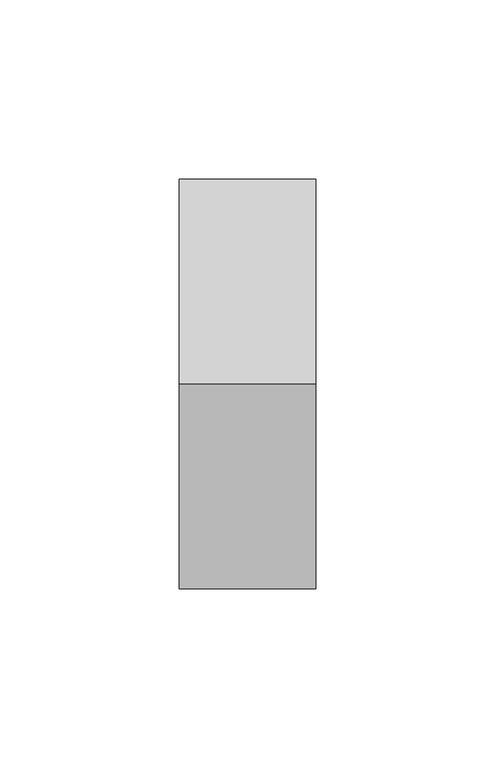
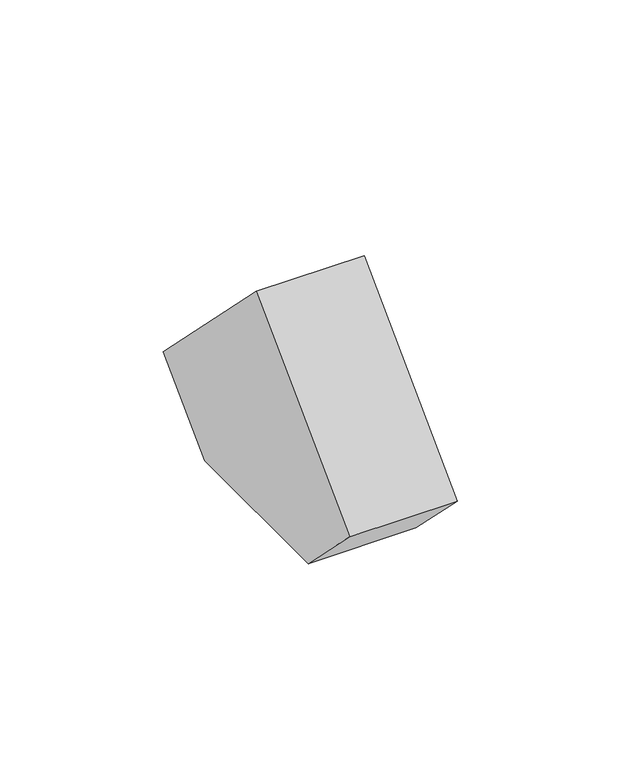
"""IFC4 building model written with IfcOpenShell, lengths in millimetres: proxy geometry, Inner panel:Inner panel:1:Inner panel:1 : Inner panel:Inner panel:300324:2:Inner panel:1:Inner panel:1 : Inner panel:Inner panel:300324:2 : Inner panel:Inner panel:1:Inner panel:1 : Inner panel:Inner panel:300324:300043:2 : Inner panel:Inner panel:1:Inner panel:1 : Inner panel:Inner panel:300324:2:Inner panel:1:Inner panel:1 : Inner panel:Inner panel:300324:2 : Inner panel:Inner panel:1:Inner panel:1 : Inner panel:Inner panel:300324:300043:308120."""

from ifc_helpers import new_model, si_unit, frame, origin, place, context, project, spatial, polyline, outline, extrude, source, transform, mapped, element, save


def generic_models_094954bc(model_context):
    return source(origin(), model_context, "Body", "SweptSolid", [
        extrude(outline(polyline([(-569594.8513281, 8849.4498692), (-569620.2513282, 8824.0498691), (-569683.7513282, 8824.0498691), (-569709.1513281, 8849.4498691), (-569652.0013281, 8906.5998691), (-569594.8513281, 8849.4498692)])), frame((593426.9367239, 0.0, 0.0), z_axis=(1.0, 0.0, 0.0), x_axis=(0.0, 1.0, 0.0)), (0.0, 0.0, 1.0), 38.1),
    ])


if __name__ == "__main__":
    model = new_model("IFC4")
    model_context = context("Model", 3, world=origin())
    ifc_project = project(units=[si_unit("LENGTHUNIT", "METRE", prefix="MILLI")], contexts=[model_context])
    site = spatial("IfcSite", under=ifc_project)
    building = spatial("IfcBuilding", under=site)
    placement = place(None, origin())
    generic_models_shape = generic_models_094954bc(model_context)
    element("IfcBuildingElementProxy", 1, Name="Inner panel:Inner panel:1:Inner panel:1 : Inner panel:Inner panel:300324:2:Inner panel:1:Inner panel:1 : Inner panel:Inner panel:300324:2 : Inner panel:Inner panel:1:Inner panel:1 : Inner panel:Inner panel:300324:300043:2 : Inner panel:Inner panel:1:Inner panel:1 : Inner panel:Inner panel:300324:2:Inner panel:1:Inner panel:1 : Inner panel:Inner panel:300324:2 : Inner panel:Inner panel:1:Inner panel:1 : Inner panel:Inner panel:300324:300043:308120", ObjectType="Inner panel:Inner panel:1:Inner panel:1 : Inner panel:Inner panel:300324:2:Inner panel:1:Inner panel:1 : Inner panel:Inner panel:300324:2 : Inner panel:Inner panel:1:Inner panel:1 : Inner panel:Inner panel:300324:300043:2 : Inner panel:Inner panel:1:Inner panel:1 : Inner panel:Inner panel:300324:2:Inner panel:1:Inner panel:1 : Inner panel:Inner panel:300324:2 : Inner panel:Inner panel:1:Inner panel:1 : Inner panel:Inner panel:300324:300043:308120", at=placement, inside=building, context=model_context, shape_type="MappedRepresentation", body=[
        mapped(generic_models_shape, transform((0.0, 0.0, 0.0), x_axis=(1.0, 0.0, 0.0), y_axis=(0.0, 1.0, 0.0), z_axis=(0.0, 0.0, 1.0))),
    ])
    save(model, "model.ifc")

# Revit data of these elements
# Type "Inner panel:Inner panel:1:Inner panel:1 : Inner panel:Inner panel:300324:2:Inner panel:1:Inner panel:1 : Inner panel:Inner panel:300324:2 : Inner panel:Inner panel:1:Inner panel:1 : Inner panel:Inner panel:300324:300043:2 : Inner panel:Inner panel:1:Inner panel:1 : Inner panel:Inner panel:300324:2:Inner panel:1:Inner panel:1 : Inner panel:Inner panel:300324:2 : Inner panel:Inner panel:1:Inner panel:1 : Inner panel:Inner panel:300324:300043:308120"
#   NameOverride = "Inner panel:Inner panel:1:Inner panel:1 : Inner panel:Inner panel:300324:2:Inner panel:1:Inner panel:1 : Inner panel:Inner panel:300324:2 : Inner panel:Inner panel:1:Inner panel:1 : Inner panel:Inner panel:300324:300043:308120"
#   ObjectTypeOverride = "Inner panel:1:Inner panel:1 : Inner panel:Inner panel:300324:2 : Inner panel:Inner panel:1:Inner panel:1 : Inner panel:Inner panel:300324:300043"
#   Reference = "Inner panel"
#   Tag = "308120"
# Element 1 (IfcBuildingElementProxy, "Inner panel:Inner panel:1:Inner panel:1 : Inner panel:Inner panel:300324:2:Inner panel:1:Inner panel:1 : Inner panel:Inner panel:300324:2 : Inner panel:Inner panel:1:Inner panel:1 : Inner panel:Inner panel:300324:300043:2 : Inner panel:Inner panel:1:Inner panel:1 : Inner panel:Inner panel:300324:2:Inner panel:1:Inner panel:1 : Inner panel:Inner panel:300324:2 : Inner panel:Inner panel:1:Inner panel:1 : Inner panel:Inner panel:300324:300043:308120")
#   Materials on its faces: "SNOW GUARD SYSTEM"
# Materials
#   "SNOW GUARD SYSTEM": class "Generic", colour RGB 223 223 223, transparency 0, Cost = 0
